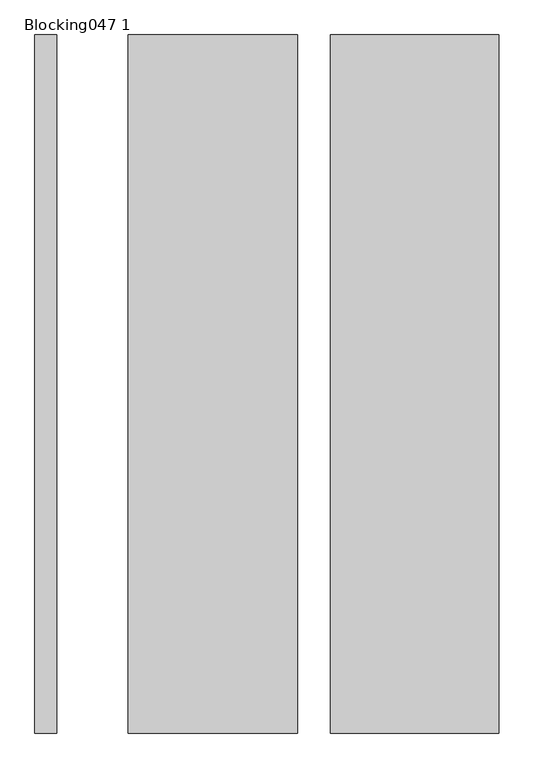
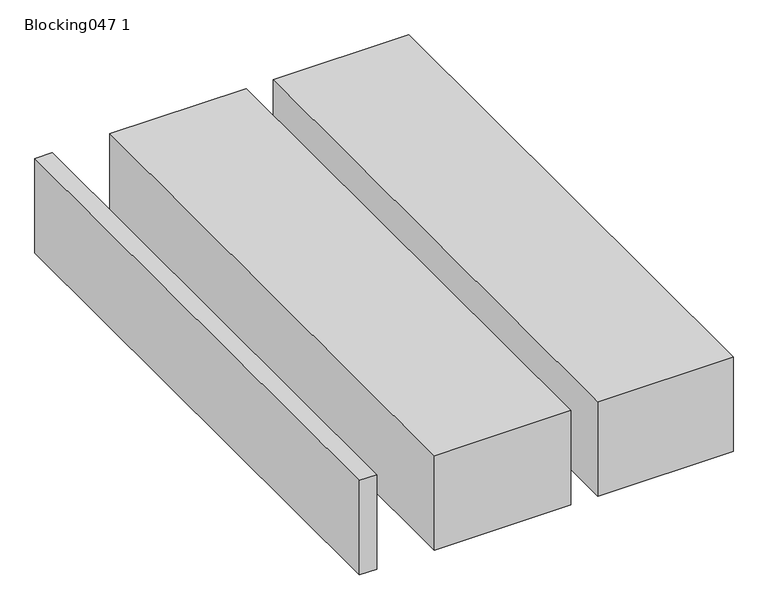
"""IFC4 building model written with IfcOpenShell, lengths in millimetres: proxy geometry, Blocking047 1 : Blocking047 2889."""

from ifc_helpers import new_model, si_unit, frame, origin, place, context, project, spatial, polyline, outline, extrude, source, transform, mapped, element, save


def blocking047_1_652cf5f5(model_context):
    return source(origin(), model_context, "Body", "SweptSolid", [
        extrude(outline(polyline([(-1224.0231587, -1052.8908936), (-1706.6231587, -1052.8908936), (-1706.6231587, 947.1091064), (-1224.0231587, 947.1091064), (-1224.0231587, -1052.8908936)])), frame((0.0, 0.0, 39744.3947923), z_axis=(0.0, 0.0, 1.0), x_axis=(1.0, 0.0, 0.0)), (0.0, 0.0, 1.0), 355.6),
        extrude(outline(polyline([(-1802.0706359, -1052.8908936), (-2287.3302122, -1052.8908936), (-2287.3302122, 947.1091064), (-1802.0706359, 947.1091064), (-1802.0706359, -1052.8908936)])), frame((0.0, 0.0, 39744.3947923), z_axis=(0.0, 0.0, 1.0), x_axis=(1.0, 0.0, 0.0)), (0.0, 0.0, 1.0), 355.6),
        extrude(outline(polyline([(-2492.5394872, -1052.8908936), (-2554.5871821, -1052.8908936), (-2554.5871821, 947.1091064), (-2492.5394872, 947.1091064), (-2492.5394872, -1052.8908936)])), frame((0.0, 0.0, 39744.3947923), z_axis=(0.0, 0.0, 1.0), x_axis=(1.0, 0.0, 0.0)), (0.0, 0.0, 1.0), 355.6),
    ])


if __name__ == "__main__":
    model = new_model("IFC4")
    model_context = context("Model", 3, world=origin())
    ifc_project = project(units=[si_unit("LENGTHUNIT", "METRE", prefix="MILLI")], contexts=[model_context])
    site = spatial("IfcSite", under=ifc_project)
    building = spatial("IfcBuilding", under=site)
    placement = place(None, origin())
    blocking047_1_shape = blocking047_1_652cf5f5(model_context)
    element("IfcBuildingElementProxy", 1, Name="Blocking047 1 : Blocking047 2889", ObjectType="Blocking047 1 : Blocking047 2889", at=placement, inside=building, context=model_context, shape_type="MappedRepresentation", body=[
        mapped(blocking047_1_shape, transform((0.0, 0.0, 0.0), x_axis=(1.0, 0.0, 0.0), y_axis=(0.0, 1.0, 0.0), z_axis=(0.0, 0.0, 1.0))),
    ])
    save(model, "model.ifc")

# Revit data of these elements
# Type "Blocking047 1 : Blocking047 2889"
#   NameOverride = "Blocking047"
# Element 1 (IfcBuildingElementProxy, "Blocking047 1 : Blocking047 2889")
#   Materials on its faces: "BATT INSULATION AT CEILING/ROOF (R-FACTOR = R30 MIN) OVER CLASS II VAPOR RETARDER (TOWARD INTERIOR)"
# Materials
#   "BATT INSULATION AT CEILING/ROOF (R-FACTOR = R30 MIN) OVER CLASS II VAPOR RETARDER (TOWARD INTERIOR)": class "Unassigned", colour RGB 245 226 176, transparency 0, Cost = 0
